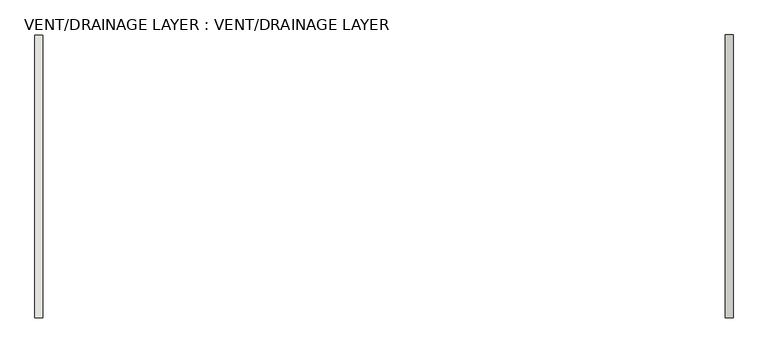
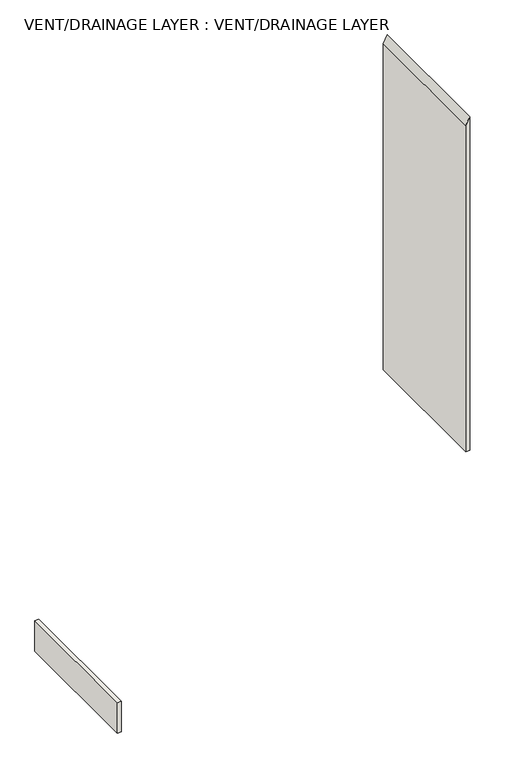
"""IFC4 building model written with IfcOpenShell, lengths in millimetres: wall geometry, VENT/DRAINAGE LAYER : VENT/DRAINAGE LAYER."""

from ifc_helpers import new_model, si_unit, frame, origin, place, context, project, spatial, polyline, outline, extrude, source, transform, mapped, element, save


def vent_drainage_layer_vent_drainage_layer_9036c45d(model_context):
    return source(origin(), model_context, "Body", "SweptSolid", [
        extrude(outline(polyline([(17915.1315703, -2319.6634634), (17896.0815703, -2319.6634634), (17896.0815703, -1633.8634634), (17915.1315703, -1633.8634634), (17915.1315703, -2319.6634634)])), frame((0.0, 0.0, 2198.6875), z_axis=(0.0, 0.0, 1.0), x_axis=(1.0, 0.0, 0.0)), (0.0, 0.0, 1.0), 154.9707982),
        extrude(outline(polyline([(4699.3557155, 19570.3024835), (3041.7352617, 19570.3024835), (3041.7352617, 19589.3538317), (4737.4584118, 19589.3538317), (4699.3557155, 19570.3024835)])), frame((0.0, -2319.6634634, 0.0), z_axis=(0.0, 1.0, 0.0), x_axis=(0.0, 0.0, 1.0)), (0.0, 0.0, 1.0), 685.8),
    ])


if __name__ == "__main__":
    model = new_model("IFC4")
    model_context = context("Model", 3, world=origin())
    ifc_project = project(units=[si_unit("LENGTHUNIT", "METRE", prefix="MILLI")], contexts=[model_context])
    site = spatial("IfcSite", under=ifc_project)
    building = spatial("IfcBuilding", under=site)
    placement = place(None, origin())
    vent_drainage_layer_vent_drainage_layer_shape = vent_drainage_layer_vent_drainage_layer_9036c45d(model_context)
    element("IfcWall", 1, ObjectType="VENT/DRAINAGE LAYER : VENT/DRAINAGE LAYER", at=placement, inside=building, context=model_context, shape_type="MappedRepresentation", body=[
        mapped(vent_drainage_layer_vent_drainage_layer_shape, transform((0.0, 0.0, 0.0), x_axis=(1.0, 0.0, 0.0), y_axis=(0.0, 1.0, 0.0), z_axis=(0.0, 0.0, 1.0))),
    ])
    save(model, "model.ifc")

# Revit data of these elements
# Element 1 (IfcWall, "VENT/DRAINAGE LAYER : VENT/DRAINAGE LAYER")
#   Materials on its faces: "VENT/DRAINAGE LAYER"
# Materials
#   "VENT/DRAINAGE LAYER": class "Miscellaneous", colour RGB 127 127 127, transparency 0, Cost = 0
